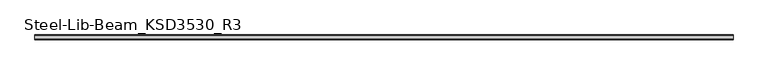
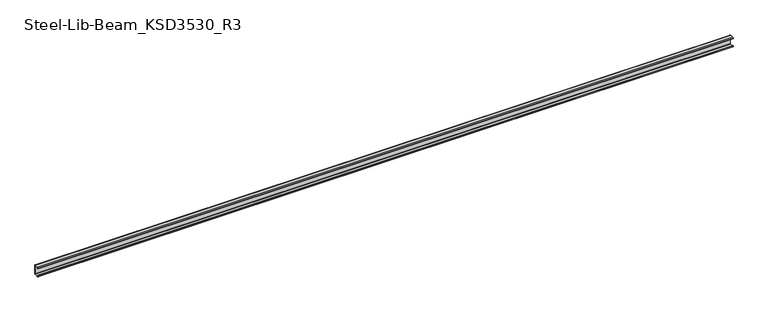
"""IFC4 building model written with IfcOpenShell, lengths in millimetres: beam geometry, Steel-Lib-Beam_KSD3530_R3 : BMS291_C-150×75x20x4.5."""

from ifc_helpers import new_model, si_unit, point, frame, frame_2d, origin, place, context, project, spatial, polyline, circle_curve, trimmed, segment, composite_curve, outline, extrude, source, transform, mapped, element, save


def steel_lib_beam_ksd3530_r3_c3d30319(model_context):
    return source(origin(), model_context, "Body", "SweptSolid", [
        extrude(outline(composite_curve([segment(trimmed(circle_curve(frame_2d((-41.0, 66.0)), 9.0), [point((-50.0, 66.0))], [point((-41.0, 75.0))], False, "CARTESIAN"), True, "CONTINUOUS"), segment(polyline([(-41.0, 75.0), (16.0, 75.0)]), True, "CONTINUOUS"), segment(trimmed(circle_curve(frame_2d((16.0, 66.0)), 9.0), [point((16.0, 75.0))], [point((25.0, 66.0))], False, "CARTESIAN"), True, "CONTINUOUS"), segment(polyline([(25.0, 66.0), (25.0, -66.0)]), True, "CONTINUOUS"), segment(trimmed(circle_curve(frame_2d((16.0, -66.0)), 9.0), [point((25.0, -66.0))], [point((16.0, -75.0))], False, "CARTESIAN"), True, "CONTINUOUS"), segment(polyline([(16.0, -75.0), (-41.0, -75.0)]), True, "CONTINUOUS"), segment(trimmed(circle_curve(frame_2d((-41.0, -66.0)), 9.0), [point((-41.0, -75.0))], [point((-50.0, -66.0))], False, "CARTESIAN"), True, "CONTINUOUS"), segment(polyline([(-50.0, -66.0), (-50.0, -55.0), (-45.5, -55.0), (-45.5, -66.0)]), True, "CONTINUOUS"), segment(trimmed(circle_curve(frame_2d((-41.0, -66.0)), 4.5), [point((-45.5, -66.0))], [point((-41.0, -70.5))], True, "CARTESIAN"), True, "CONTINUOUS"), segment(polyline([(-41.0, -70.5), (16.0, -70.5)]), True, "CONTINUOUS"), segment(trimmed(circle_curve(frame_2d((16.0, -66.0)), 4.5), [point((16.0, -70.5))], [point((20.5, -66.0))], True, "CARTESIAN"), True, "CONTINUOUS"), segment(polyline([(20.5, -66.0), (20.5, 66.0)]), True, "CONTINUOUS"), segment(trimmed(circle_curve(frame_2d((16.0, 66.0)), 4.5), [point((20.5, 66.0))], [point((16.0, 70.5))], True, "CARTESIAN"), True, "CONTINUOUS"), segment(polyline([(16.0, 70.5), (-41.0, 70.5)]), True, "CONTINUOUS"), segment(trimmed(circle_curve(frame_2d((-41.0, 66.0)), 4.5), [point((-41.0, 70.5))], [point((-45.5, 66.0))], True, "CARTESIAN"), True, "CONTINUOUS"), segment(polyline([(-45.5, 66.0), (-45.5, 55.0), (-50.0, 55.0), (-50.0, 66.0)]), True, "CONTINUOUS")], self_intersect=False)), frame((-5290.0, 0.0, 0.0), z_axis=(1.0, 0.0, 0.0), x_axis=(0.0, 1.0, 0.0)), (0.0, 0.0, 1.0), 10580.0),
    ])


if __name__ == "__main__":
    model = new_model("IFC4")
    model_context = context("Model", 3, world=origin())
    ifc_project = project(units=[si_unit("LENGTHUNIT", "METRE", prefix="MILLI")], contexts=[model_context])
    site = spatial("IfcSite", under=ifc_project)
    building = spatial("IfcBuilding", under=site)
    placement = place(None, origin())
    steel_lib_beam_ksd3530_r3_shape = steel_lib_beam_ksd3530_r3_c3d30319(model_context)
    element("IfcBeam", 1, ObjectType="Steel-Lib-Beam_KSD3530_R3 : BMS291_C-150×75x20x4.5", at=placement, inside=building, context=model_context, shape_type="MappedRepresentation", body=[
        mapped(steel_lib_beam_ksd3530_r3_shape, transform((0.0, 0.0, 0.0), x_axis=(1.0, 0.0, 0.0), y_axis=(0.0, 1.0, 0.0), z_axis=(0.0, 0.0, 1.0))),
    ])
    save(model, "model.ifc")

# Revit data of these elements
# Type "Steel-Lib-Beam_KSD3530_R3 : BMS291_C-150×75x20x4.5"
#   Keynote = "C-150×75x20x4.5"
#   SteelWeight = "Light"
#   x = 0.0250 m
#   t1 = 0.0090 m
#   t = 0.0045 m
#   Surface Area = 0.629834 m²/m
#   Section Area = 13.9688 cm²
#   Mass per Unit Length = 10.9655 kg/m
#   C = 0.0200 m
#   A = 0.0750 m
#   Length [instance default] = 1.5000 m
#   H = 0.1500 m
#   hec_material4 [instance default] = none
#   hec_material3 [instance default] = none
#   hec_material2 [instance default] = none
#   hec_material1 [instance default] = none
#   Structural Material [instance default] = Metal - Steel - Light Gauge
#   Assembly Code = ""
# Element 1 (IfcBeam, "Steel-Lib-Beam_KSD3530_R3 : BMS291_C-150×75x20x4.5")
#   Structural Material = none
# Materials
#   "Metal - Steel - Light Gauge": class "Metal", colour RGB 247 247 247, transparency 0
